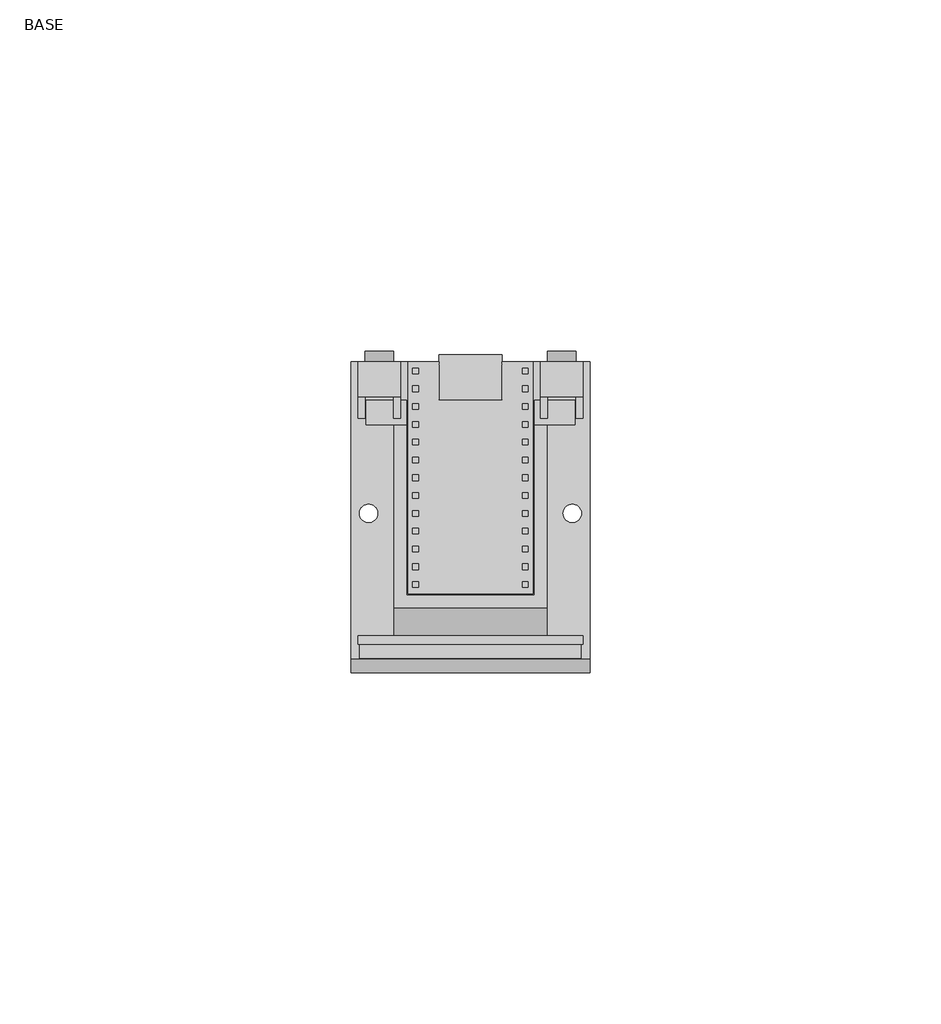
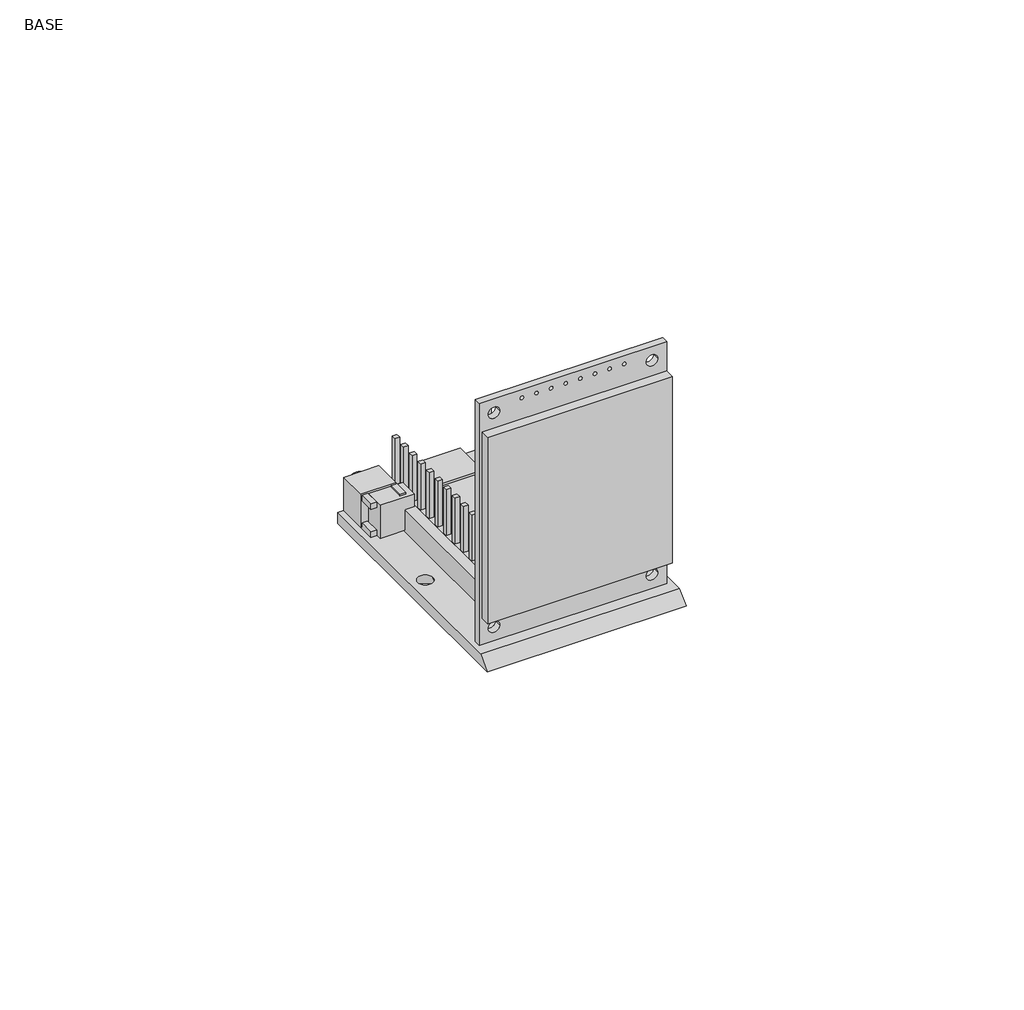
# One storey: 4 furniture elements, 1 proxy.
# Revit data of these elements (continued)
# Materials (continued)
#   ".VIDRO": class "Vidro", colour RGB 165 190 164, transparency 0.4, Cost = 0
#   ".CHIP": class "Vidro", colour RGB 236 240 239, transparency 0.35, Cost = 0
#   ".BOTAO": class "Vidro", colour RGB 0 255 255, transparency 0.75, Cost = 0
